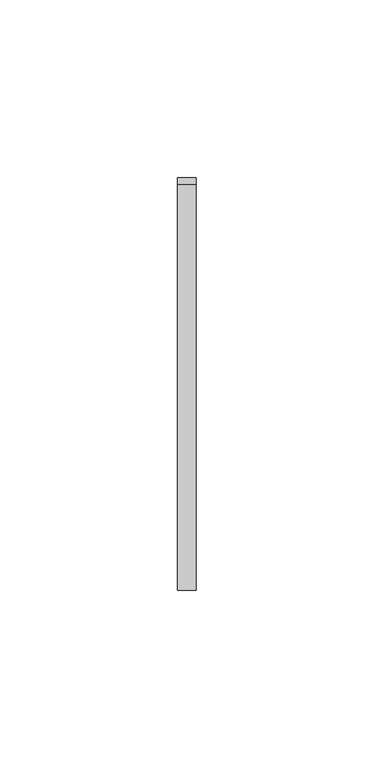
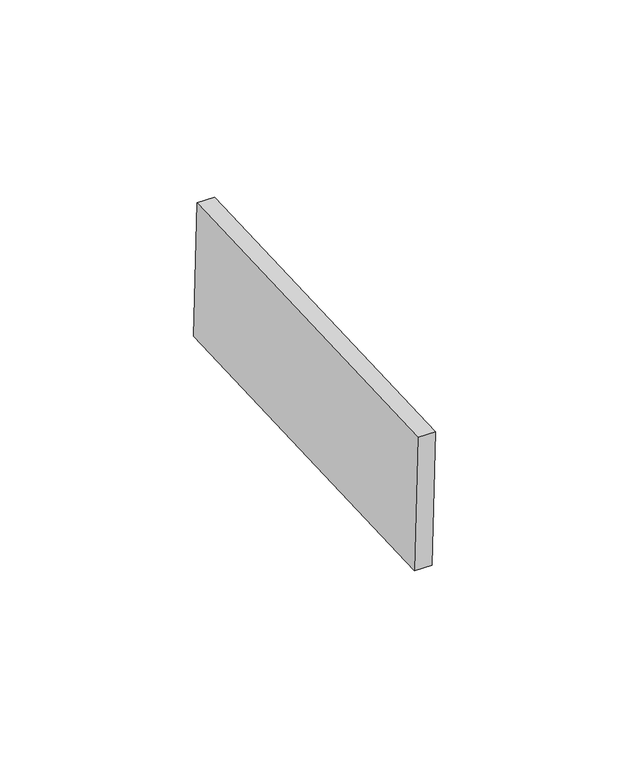
"""IFC4 building model written with IfcOpenShell, lengths in millimetres: proxy geometry, Inner panel:Inner panel:1:Inner panel:1 : Inner panel:Inner panel:300324:2:Inner panel:1:Inner panel:1 : Inner panel:Inner panel:300324:2 : Inner panel:Inner panel:1:Inner panel:1 : Inner panel:Inner panel:300324:300043:101 : Inner panel:Inner panel:1:Inner panel:1 : Inner panel:Inner panel:300324:2:Inner panel:1:Inner panel:1 : Inner panel:Inner panel:300324:2 : Inner panel:Inner panel:1:Inner panel:1 : Inner panel:Inner panel:300324:300043:308120."""

from ifc_helpers import new_model, si_unit, frame, origin, place, context, project, spatial, polyline, outline, extrude, source, transform, mapped, element, save


def generic_models_9287129c(model_context):
    return source(origin(), model_context, "Body", "SweptSolid", [
        extrude(outline(polyline([(0.0, -114.3), (0.0, 0.0), (5.2138089, 0.0), (5.2138089, -114.3), (0.0, -114.3)])), frame((592310.995117, -579834.7443474, 3917.6246678), z_axis=(0.0, -0.04163054471216399, 0.9991330730923527), x_axis=(-1.0, 0.0, 0.0)), (0.0, 0.0, 1.0), 43.2233908),
    ])


if __name__ == "__main__":
    model = new_model("IFC4")
    model_context = context("Model", 3, world=origin())
    ifc_project = project(units=[si_unit("LENGTHUNIT", "METRE", prefix="MILLI")], contexts=[model_context])
    site = spatial("IfcSite", under=ifc_project)
    building = spatial("IfcBuilding", under=site)
    placement = place(None, origin())
    generic_models_shape = generic_models_9287129c(model_context)
    element("IfcBuildingElementProxy", 1, Name="Inner panel:Inner panel:1:Inner panel:1 : Inner panel:Inner panel:300324:2:Inner panel:1:Inner panel:1 : Inner panel:Inner panel:300324:2 : Inner panel:Inner panel:1:Inner panel:1 : Inner panel:Inner panel:300324:300043:101 : Inner panel:Inner panel:1:Inner panel:1 : Inner panel:Inner panel:300324:2:Inner panel:1:Inner panel:1 : Inner panel:Inner panel:300324:2 : Inner panel:Inner panel:1:Inner panel:1 : Inner panel:Inner panel:300324:300043:308120", ObjectType="Inner panel:Inner panel:1:Inner panel:1 : Inner panel:Inner panel:300324:2:Inner panel:1:Inner panel:1 : Inner panel:Inner panel:300324:2 : Inner panel:Inner panel:1:Inner panel:1 : Inner panel:Inner panel:300324:300043:101 : Inner panel:Inner panel:1:Inner panel:1 : Inner panel:Inner panel:300324:2:Inner panel:1:Inner panel:1 : Inner panel:Inner panel:300324:2 : Inner panel:Inner panel:1:Inner panel:1 : Inner panel:Inner panel:300324:300043:308120", at=placement, inside=building, context=model_context, shape_type="MappedRepresentation", body=[
        mapped(generic_models_shape, transform((0.0, 0.0, 0.0), x_axis=(1.0, 0.0, 0.0), y_axis=(0.0, 1.0, 0.0), z_axis=(0.0, 0.0, 1.0))),
    ])
    save(model, "model.ifc")

# Revit data of these elements
# Type "Inner panel:Inner panel:1:Inner panel:1 : Inner panel:Inner panel:300324:2:Inner panel:1:Inner panel:1 : Inner panel:Inner panel:300324:2 : Inner panel:Inner panel:1:Inner panel:1 : Inner panel:Inner panel:300324:300043:101 : Inner panel:Inner panel:1:Inner panel:1 : Inner panel:Inner panel:300324:2:Inner panel:1:Inner panel:1 : Inner panel:Inner panel:300324:2 : Inner panel:Inner panel:1:Inner panel:1 : Inner panel:Inner panel:300324:300043:308120"
#   NameOverride = "Inner panel:Inner panel:1:Inner panel:1 : Inner panel:Inner panel:300324:2:Inner panel:1:Inner panel:1 : Inner panel:Inner panel:300324:2 : Inner panel:Inner panel:1:Inner panel:1 : Inner panel:Inner panel:300324:300043:308120"
#   ObjectTypeOverride = "Inner panel:1:Inner panel:1 : Inner panel:Inner panel:300324:2 : Inner panel:Inner panel:1:Inner panel:1 : Inner panel:Inner panel:300324:300043"
#   Reference = "Inner panel"
#   Tag = "308120"
# Element 1 (IfcBuildingElementProxy, "Inner panel:Inner panel:1:Inner panel:1 : Inner panel:Inner panel:300324:2:Inner panel:1:Inner panel:1 : Inner panel:Inner panel:300324:2 : Inner panel:Inner panel:1:Inner panel:1 : Inner panel:Inner panel:300324:300043:101 : Inner panel:Inner panel:1:Inner panel:1 : Inner panel:Inner panel:300324:2:Inner panel:1:Inner panel:1 : Inner panel:Inner panel:300324:2 : Inner panel:Inner panel:1:Inner panel:1 : Inner panel:Inner panel:300324:300043:308120")
#   Materials on its faces: "SLIDING CLIP"
# Materials
#   "SLIDING CLIP": class "Generic", colour RGB 120 120 120, transparency 0, Cost = 0
